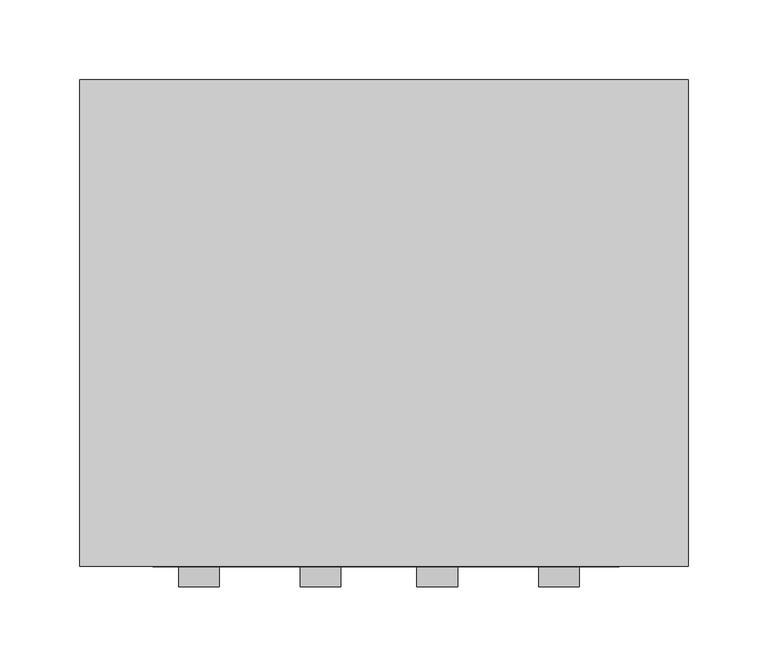
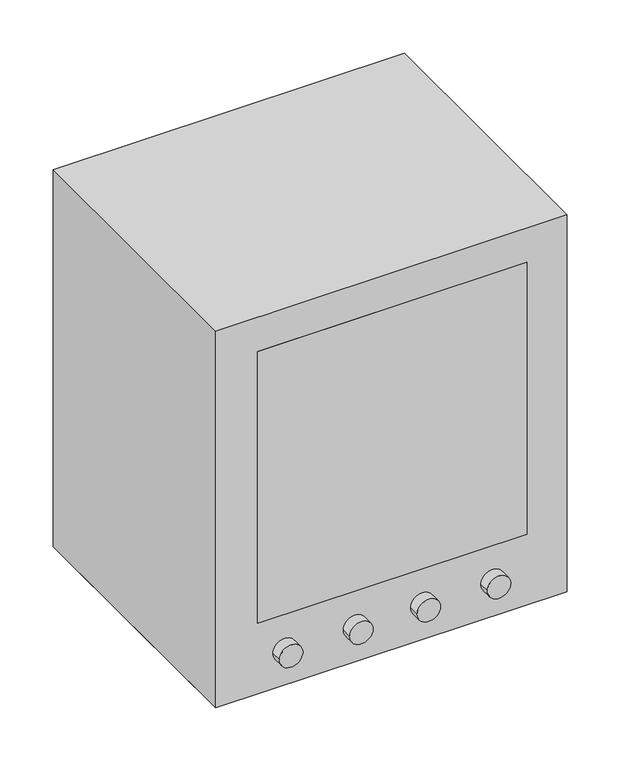
"""IFC4 building model written with IfcOpenShell, lengths in millimetres: proxy geometry, M7855 - Monitor, Physiological, Infant : M7855 - Monitor, Physiological, Infant."""

from ifc_helpers import new_model, si_unit, point, frame, frame_2d, origin, place, context, project, spatial, polyline, circle_curve, trimmed, segment, composite_curve, outline, extrude, faceted_brep, source, transform, mapped, element, save


def specialty_equipment_b5f346ec(model_context):
    return source(origin(), model_context, "Body", "SolidModel", [
        extrude(outline(polyline([(147.287649, -152.4), (-144.812351, -152.4), (-144.812351, -146.05), (147.287649, -146.05), (147.287649, -152.4)])), frame((0.0, 0.0, 81.0028485), z_axis=(0.0, 0.0, 1.0), x_axis=(1.0, 0.0, 0.0)), (0.0, 0.0, 1.0), 311.15),
        faceted_brep([(190.5, -152.4, 431.8), (-190.5, -152.4, 431.8), (-190.5, -152.4, 0.0), (190.5, -152.4, 0.0), (-144.812351, -152.4, 392.1528485), (147.287649, -152.4, 392.1528485), (147.287649, -152.4, 81.0028485), (-144.812351, -152.4, 81.0028485), (190.5, 152.4, 431.8), (190.5, 152.4, 0.0), (-190.5, 152.4, 0.0), (-190.5, 152.4, 431.8), (147.287649, -139.7, 392.1528485), (-144.812351, -139.7, 392.1528485), (-144.812351, -139.7, 81.0028485), (147.287649, -139.7, 81.0028485)], [[[0, 1, 2, 3], [4, 5, 6, 7]], [[8, 9, 10, 11]], [[1, 0, 8, 11]], [[2, 1, 11, 10]], [[3, 2, 10, 9]], [[0, 3, 9, 8]], [[12, 13, 14, 15]], [[13, 12, 5, 4]], [[14, 13, 4, 7]], [[15, 14, 7, 6]], [[12, 15, 6, 5]]]),
        faceted_brep([(-190.5, 152.4, 431.8), (-190.5, 0.0, 431.8), (-190.5, -152.4, 431.8), (190.5, -152.4, 431.8), (190.5, 152.4, 431.8), (-190.5, 152.4, 0.0), (190.5, 152.4, 0.0), (190.5, -152.4, 0.0), (-190.5, -152.4, 0.0), (-190.5, 0.0, 0.0), (-144.812351, -152.4, 392.1528485), (147.287649, -152.4, 392.1528485), (147.287649, -152.4, 81.0028485), (-144.812351, -152.4, 81.0028485), (147.287649, -139.7, 392.1528485), (-144.812351, -139.7, 392.1528485), (-144.812351, -139.7, 81.0028485), (147.287649, -139.7, 81.0028485)], [[[0, 1, 2, 3, 4]], [[5, 6, 7, 8, 9]], [[1, 0, 5, 9]], [[2, 1, 9, 8]], [[3, 2, 8, 7], [10, 11, 12, 13]], [[4, 3, 7, 6]], [[0, 4, 6, 5]], [[14, 15, 16, 17]], [[15, 14, 11, 10]], [[16, 15, 10, 13]], [[17, 16, 13, 12]], [[14, 17, 12, 11]]]),
        extrude(outline(composite_curve([segment(trimmed(circle_curve(frame_2d((41.1587525, 33.3616492)), 12.7), [point((41.1587525, 46.0616492))], [point((41.1587525, 20.6616492))], False, "CARTESIAN"), True, "CONTINUOUS"), segment(trimmed(circle_curve(frame_2d((41.1587525, 33.3616492)), 12.7), [point((41.1587525, 20.6616492))], [point((41.1587525, 46.0616492))], False, "CARTESIAN"), True, "CONTINUOUS")], self_intersect=False)), frame((0.0, -165.1, 0.0), z_axis=(0.0, 1.0, 0.0), x_axis=(0.0, 0.0, 1.0)), (0.0, 0.0, 1.0), 12.7),
        extrude(outline(composite_curve([segment(trimmed(circle_curve(frame_2d((41.1587525, 109.5616492)), 12.7), [point((41.1587525, 122.2616492))], [point((41.1587525, 96.8616492))], False, "CARTESIAN"), True, "CONTINUOUS"), segment(trimmed(circle_curve(frame_2d((41.1587525, 109.5616492)), 12.7), [point((41.1587525, 96.8616492))], [point((41.1587525, 122.2616492))], False, "CARTESIAN"), True, "CONTINUOUS")], self_intersect=False)), frame((0.0, -165.1, 0.0), z_axis=(0.0, 1.0, 0.0), x_axis=(0.0, 0.0, 1.0)), (0.0, 0.0, 1.0), 12.7),
        extrude(outline(composite_curve([segment(trimmed(circle_curve(frame_2d((41.1587525, -39.7116492)), 12.7), [point((41.1587525, -52.4116492))], [point((41.1587525, -27.0116492))], False, "CARTESIAN"), True, "CONTINUOUS"), segment(trimmed(circle_curve(frame_2d((41.1587525, -39.7116492)), 12.7), [point((41.1587525, -27.0116492))], [point((41.1587525, -52.4116492))], False, "CARTESIAN"), True, "CONTINUOUS")], self_intersect=False)), frame((0.0, -165.1, 0.0), z_axis=(0.0, 1.0, 0.0), x_axis=(0.0, 0.0, 1.0)), (0.0, 0.0, 1.0), 12.7),
        extrude(outline(composite_curve([segment(trimmed(circle_curve(frame_2d((41.1587525, -115.9116492)), 12.7), [point((41.1587525, -128.6116492))], [point((41.1587525, -103.2116492))], False, "CARTESIAN"), True, "CONTINUOUS"), segment(trimmed(circle_curve(frame_2d((41.1587525, -115.9116492)), 12.7), [point((41.1587525, -103.2116492))], [point((41.1587525, -128.6116492))], False, "CARTESIAN"), True, "CONTINUOUS")], self_intersect=False)), frame((0.0, -165.1, 0.0), z_axis=(0.0, 1.0, 0.0), x_axis=(0.0, 0.0, 1.0)), (0.0, 0.0, 1.0), 12.7),
    ])


if __name__ == "__main__":
    model = new_model("IFC4")
    model_context = context("Model", 3, world=origin())
    ifc_project = project(units=[si_unit("LENGTHUNIT", "METRE", prefix="MILLI")], contexts=[model_context])
    site = spatial("IfcSite", under=ifc_project)
    building = spatial("IfcBuilding", under=site)
    placement = place(None, origin())
    specialty_equipment_shape = specialty_equipment_b5f346ec(model_context)
    element("IfcBuildingElementProxy", 1, Name="M7855 - Monitor, Physiological, Infant : M7855 - Monitor, Physiological, Infant", ObjectType="M7855 - Monitor, Physiological, Infant : M7855 - Monitor, Physiological, Infant", at=placement, inside=building, context=model_context, shape_type="MappedRepresentation", body=[
        mapped(specialty_equipment_shape, transform((0.0, 0.0, 0.0), x_axis=(1.0, 0.0, 0.0), y_axis=(0.0, 1.0, 0.0), z_axis=(0.0, 0.0, 1.0))),
    ])
    save(model, "model.ifc")

# Revit data of these elements
# Project information
#   Room Abbreviation = "NYNN1"
#   Room Description = "Nursery, Level 1 (NYNN1)"
#   Sheets - Total = "5"
#   Project Issue Date = "Issue Date"
#   Project Status = "Project Status"
#   Client Name = "Owner"
#   Project Address = "Enter address here"
#   Project Name = "Project Name"
#   Project Number = "Project Number"
#   Publication Date = "30-Jan-15"
# Type "M7855 - Monitor, Physiological, Infant : M7855 - Monitor, Physiological, Infant"
#   Watts2 = "0"
#   Watts1 = "240"
#   Unit_Issue = "EA"
#   UTIL_6_Misc = "-"
#   UTIL_5_NonMedGas = "-"
#   UTIL_4_MiscGas = "-"
#   UTIL_3_MedGas = "-"
#   UTIL_2_Elec = "A"
#   UTIL_1_WaterDrain = "-"
#   Nomenclature = "Monitor, Physiological, Infant"
#   NSN = "6515"
#   Location [instance default] = ""
#   JSN = "M7855"
#   Fund_Source_VA = "-"
#   Fund_Source_Navy = "-"
#   Fund_Source_Army = "-"
#   Fund_Source_AF = "-"
#   ELEC_Volts2 = "0"
#   ELEC_Volts1 = "120"
#   ELEC_Phase2 = "0"
#   ELEC_Phase1 = "1"
#   ELEC_HertzSwitch = "0"
#   ELEC_HertzDependent = "-1"
#   ELEC_Hertz = "60"
#   ELEC_Amps2 = "0"
#   ELEC_Amps1 = "2"
#   DetailDescription = "Infant physiological monitor. Unit consists of blood pressure, ECG, respiration amplifier and temperature display. Used to monitor infants vital signs such as heart rate, temperature, respiration rate and oxygen saturation. Optional capabilities include tissue/blood gas values."
#   CAT_VA = "C"
#   CAT_Navy = "C"
#   CAT_IHS = "-"
#   CAT_Army = "C"
#   CAT_AF = "C"
#   BTUperhour = "0"
#   Weight_IP = 18
#   DIM_Width_IP = 1' - 3"
#   DIM_Height_IP = 1' - 5"
#   DIM_Depth_IP = 1' - 0"
# Element 1 (IfcBuildingElementProxy, "M7855 - Monitor, Physiological, Infant : M7855 - Monitor, Physiological, Infant")
#   Materials on its faces: "EquipSpace", "Glass"
# Materials
#   "EquipSpace": class "Unassigned", colour RGB 221 217 195, transparency 0.5
#   "Glass": class "Glass", colour RGB 0 128 192, transparency 0.75
